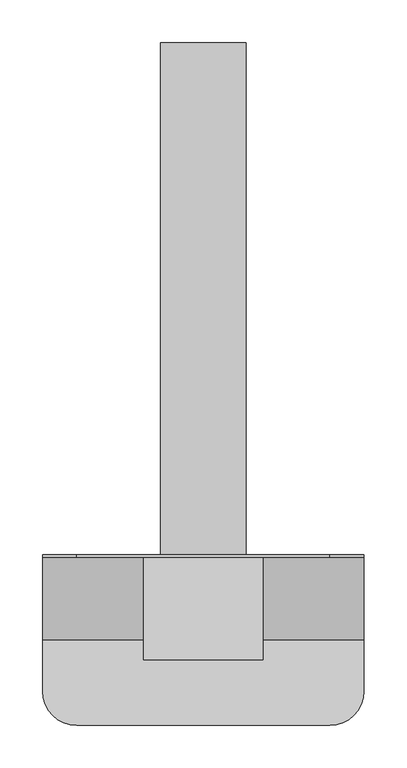
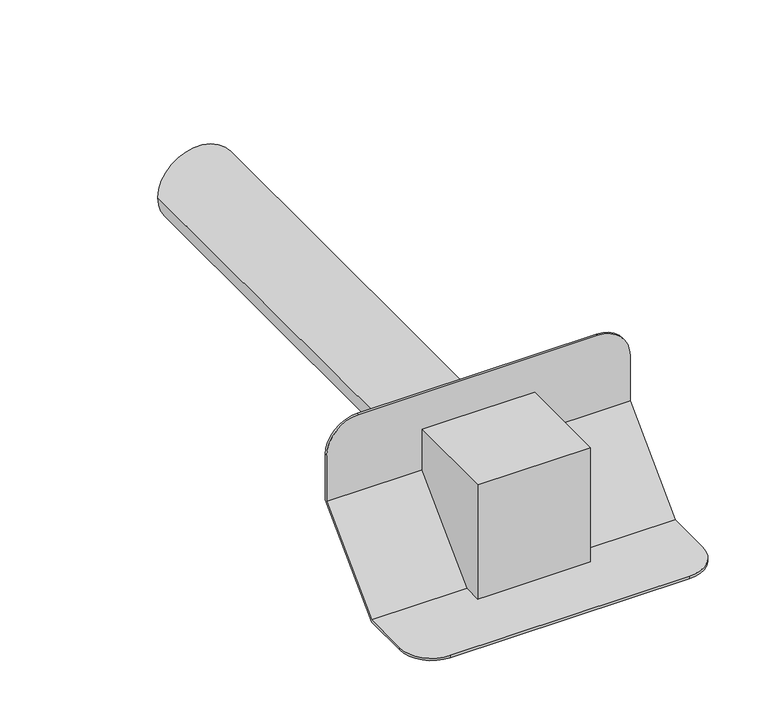
"""IFC4 building model written with IfcOpenShell, lengths in millimetres: proxy geometry, TN_Воронка парапетная ТехноНИКОЛЬ круглая_Тип 2 : Воронка парапетная ТехноНИКОЛЬ с галтелью 110х600."""

from ifc_helpers import new_model, si_unit, frame, origin, place, context, project, spatial, polyline, circle_curve, ellipse_curve, outline, extrude, source, transform, mapped, element, save
from ifc_brep_helpers import plane_surface, cylinder_surface, revolved_surface, advanced_brep


def specialty_equipment_09305b09(model_context):
    return source(origin(), model_context, "Body", "SolidModel", [
        extrude(outline(polyline([(-123.0, 3.0), (-123.0, 153.0), (-3.0, 153.0), (-3.0, 100.0), (-100.0, 3.0), (-123.0, 3.0)])), frame((-70.0, 0.0, 0.0), z_axis=(1.0, 0.0, 0.0), x_axis=(0.0, 1.0, 0.0)), (0.0, 0.0, 1.0), 140.0),
        advanced_brep(
        [(-188.5, -160.0, 3.0), (-148.5, -200.0, 3.0), (148.5, -200.0, 3.0), (188.5, -160.0, 3.0), (188.5, -100.0, 3.0), (-188.5, -100.0, 3.0), (-188.5, -160.0, 0.0), (-188.5, -100.0, 0.0), (188.5, -100.0, 0.0), (188.5, -160.0, 0.0), (148.5, -200.0, 0.0), (-148.5, -200.0, 0.0), (188.5, 0.0, 100.0), (188.5, 0.0, 160.0), (188.5, -3.0, 160.0), (188.5, -3.0, 100.0), (-188.5, -3.0, 100.0), (-188.5, -3.0, 160.0), (-188.5, 0.0, 160.0), (-188.5, 0.0, 100.0), (148.5, -3.0, 200.0), (-148.5, -3.0, 200.0), (-44.5421149, -3.0, 100.0), (44.5421149, -3.0, 100.0), (-148.5, 0.0, 200.0), (148.5, 0.0, 200.0), (47.6969601, 0.0, 100.0), (-47.6969601, 0.0, 100.0), (-50.0, 600.0, 85.0), (50.0, 600.0, 85.0), (-47.0, 600.0, 85.0), (47.0, 600.0, 85.0), (50.0, -15.0, 85.0), (-50.0, -15.0, 85.0), (47.0, -18.0, 85.0), (-47.0, -18.0, 85.0)],
        [
            (0, 1, circle_curve(frame((-148.5, -160.0, 3.0), z_axis=(0.0, 0.0, 1.0), x_axis=(1.0, 0.0, 0.0)), 40.0)),
            (1, 2),
            (2, 3, circle_curve(frame((148.5, -160.0, 3.0), z_axis=(0.0, 0.0, 1.0), x_axis=(1.0, 0.0, 0.0)), 40.0)),
            (3, 4),
            (4, 5),
            (5, 0),
            (6, 7),
            (7, 8),
            (8, 9),
            (9, 10, circle_curve(frame((148.5, -160.0, 0.0), z_axis=(0.0, 0.0, -1.0), x_axis=(1.0, 0.0, 0.0)), 40.0)),
            (10, 11),
            (11, 6, circle_curve(frame((-148.5, -160.0, 0.0), z_axis=(0.0, 0.0, -1.0), x_axis=(1.0, 0.0, 0.0)), 40.0)),
            (0, 6),
            (11, 1),
            (10, 2),
            (9, 3),
            (8, 12),
            (12, 13),
            (13, 14),
            (14, 15),
            (15, 4),
            (5, 16),
            (16, 17),
            (17, 18),
            (18, 19),
            (19, 7),
            (14, 20, circle_curve(frame((148.5, -3.0, 160.0), z_axis=(0.0, -1.0, 0.0), x_axis=(1.0, 0.0, 0.0)), 40.0)),
            (20, 21),
            (21, 17, circle_curve(frame((-148.5, -3.0, 160.0), z_axis=(0.0, -1.0, 0.0), x_axis=(1.0, 0.0, 0.0)), 40.0)),
            (16, 22),
            (22, 23, circle_curve(frame((0.0, -3.0, 85.0), z_axis=(0.0, 1.0, 0.0), x_axis=(1.0, 0.0, 0.0)), 47.0)),
            (23, 15),
            (18, 24, circle_curve(frame((-148.5, 0.0, 160.0), z_axis=(0.0, 1.0, 0.0), x_axis=(1.0, 0.0, 0.0)), 40.0)),
            (24, 25),
            (25, 13, circle_curve(frame((148.5, 0.0, 160.0), z_axis=(0.0, 1.0, 0.0), x_axis=(1.0, 0.0, 0.0)), 40.0)),
            (12, 26),
            (26, 27, circle_curve(frame((0.0, 0.0, 85.0), z_axis=(0.0, -1.0, 0.0), x_axis=(1.0, 0.0, 0.0)), 50.0)),
            (27, 19),
            (25, 20),
            (24, 21),
            (28, 29, circle_curve(frame((0.0, 600.0, 85.0), z_axis=(0.0, 1.0, 0.0), x_axis=(1.0, 0.0, 0.0)), 50.0)),
            (29, 28, circle_curve(frame((0.0, 600.0, 85.0), z_axis=(0.0, 1.0, 0.0), x_axis=(1.0, 0.0, 0.0)), 50.0)),
            (30, 31, circle_curve(frame((0.0, 600.0, 85.0), z_axis=(0.0, -1.0, 0.0), x_axis=(1.0, 0.0, 0.0)), 47.0)),
            (31, 30, circle_curve(frame((0.0, 600.0, 85.0), z_axis=(0.0, -1.0, 0.0), x_axis=(1.0, 0.0, 0.0)), 47.0)),
            (29, 32),
            (32, 33, ellipse_curve(frame((0.0, -15.0, 85.0), z_axis=(0.0, 0.7071067811865469, -0.7071067811865481), x_axis=(0.0, -0.7071067811865481, -0.7071067811865469)), 70.7106781, 50.0)),
            (33, 28),
            (33, 27, ellipse_curve(frame((0.0, -15.0, 85.0), z_axis=(0.0, 0.7071067811865469, -0.7071067811865481), x_axis=(0.0, -0.7071067811865481, -0.7071067811865469)), 70.7106781, 50.0)),
            (26, 32, ellipse_curve(frame((0.0, -15.0, 85.0), z_axis=(0.0, 0.7071067811865469, -0.7071067811865481), x_axis=(0.0, -0.7071067811865481, -0.7071067811865469)), 70.7106781, 50.0)),
            (31, 34),
            (34, 23, ellipse_curve(frame((0.0, -18.0, 85.0), z_axis=(0.0, -0.7071067811865469, 0.7071067811865482), x_axis=(0.0, 0.707106781186548, 0.7071067811865469)), 66.4680374, 47.0)),
            (22, 35, ellipse_curve(frame((0.0, -18.0, 85.0), z_axis=(0.0, -0.7071067811865469, 0.7071067811865482), x_axis=(0.0, 0.707106781186548, 0.7071067811865469)), 66.4680374, 47.0)),
            (35, 30),
            (35, 34, ellipse_curve(frame((0.0, -18.0, 85.0), z_axis=(0.0, -0.7071067811865469, 0.7071067811865482), x_axis=(0.0, 0.707106781186548, 0.7071067811865469)), 66.4680374, 47.0)),
        ],
        [
            plane_surface(frame((-108.5, -160.0, 3.0), z_axis=(0.0, 0.0, 1.0), x_axis=(0.0, 1.0, 0.0))),
            plane_surface(frame((-108.5, -160.0, 0.0), z_axis=(0.0, 0.0, -1.0), x_axis=(0.0, -1.0, 0.0))),
            cylinder_surface(frame((-148.5, -160.0, 0.0), z_axis=(0.0, 0.0, 1.0), x_axis=(1.0, 0.0, 0.0)), 40.0),
            plane_surface(frame((-148.5, -200.0, 3.0), z_axis=(0.0, -1.0, 0.0), x_axis=(0.0, 0.0, -1.0))),
            cylinder_surface(frame((148.5, -160.0, 0.0), z_axis=(0.0, 0.0, 1.0), x_axis=(1.0, 0.0, 0.0)), 40.0),
            plane_surface(frame((188.5, -160.0, 3.0), z_axis=(1.0, 0.0, 0.0), x_axis=(0.0, 0.0, -1.0))),
            plane_surface(frame((-188.5, -100.0, 3.0), z_axis=(-1.0, 0.0, 0.0), x_axis=(0.0, 0.0, -1.0))),
            plane_surface(frame((-188.5, -3.0, 100.0), z_axis=(0.0, -1.0, 0.0), x_axis=(1.0, 0.0, 0.0))),
            plane_surface(frame((-188.5, 0.0, 100.0), z_axis=(0.0, 1.0, 0.0), x_axis=(-1.0, 0.0, 0.0))),
            cylinder_surface(frame((148.5, 0.0, 160.0), z_axis=(0.0, -1.0, 0.0), x_axis=(1.0, 0.0, 0.0)), 40.0),
            plane_surface(frame((148.5, -3.0, 200.0), z_axis=(0.0, 0.0, 1.0), x_axis=(0.0, 1.0, 0.0))),
            cylinder_surface(frame((-148.5, 0.0, 160.0), z_axis=(0.0, -1.0, 0.0), x_axis=(1.0, 0.0, 0.0)), 40.0),
            plane_surface(frame((50.0, 600.0, 85.0), z_axis=(0.0, 1.0, 0.0), x_axis=(0.0, 0.0, -1.0))),
            cylinder_surface(frame((0.0, 600.0, 85.0), z_axis=(0.0, -1.0, 0.0), x_axis=(1.0, 0.0, 0.0)), 50.0),
            revolved_surface(polyline([(47.0, 600.0, 85.0), (47.0, -64.9999999777011, 85.0)]), (0.0, 0.0, 85.0), (0.0, 1.0, 0.0)),
            plane_surface(frame((188.5, -3.0, 100.0), z_axis=(0.0, -0.7071067811865469, 0.7071067811865482), x_axis=(-1.0, 0.0, 0.0))),
            plane_surface(frame((188.5, -100.0, 0.0), z_axis=(0.0, 0.7071067811865469, -0.7071067811865481), x_axis=(-1.0, 0.0, 0.0))),
        ],
        [
            (0, [[1, 2, 3, 4, 5, 6]]),
            (1, [[7, 8, 9, 10, 11, 12]]),
            (2, [[-1, 13, -12, 14]]),
            (3, [[-2, -14, -11, 15]]),
            (4, [[-3, -15, -10, 16]]),
            (5, [[-4, -16, -9, 17, 18, 19, 20, 21]]),
            (6, [[-6, 22, 23, 24, 25, 26, -7, -13]]),
            (7, [[-20, 27, 28, 29, -23, 30, 31, 32]]),
            (8, [[-25, 33, 34, 35, -18, 36, 37, 38]]),
            (9, [[-27, -19, -35, 39]]),
            (10, [[-28, -39, -34, 40]]),
            (11, [[-29, -40, -33, -24]]),
            (12, [[41, 42], [43, 44]]),
            (13, [[-42, 45, 46, 47]]),
            (13, [[-41, -47, 48, -37, 49, -45]]),
            (14, [[-44, 50, 51, -31, 52, 53]]),
            (14, [[-43, -53, 54, -50]]),
            (15, [[-21, -32, -51, -54, -52, -30, -22, -5]]),
            (16, [[-17, -8, -26, -38, -48, -46, -49, -36]]),
        ],
    ),
    ])


if __name__ == "__main__":
    model = new_model("IFC4")
    model_context = context("Model", 3, world=origin())
    ifc_project = project(units=[si_unit("LENGTHUNIT", "METRE", prefix="MILLI")], contexts=[model_context])
    site = spatial("IfcSite", under=ifc_project)
    building = spatial("IfcBuilding", under=site)
    placement = place(None, origin())
    specialty_equipment_shape = specialty_equipment_09305b09(model_context)
    element("IfcBuildingElementProxy", 1, Name="TN_Воронка парапетная ТехноНИКОЛЬ круглая_Тип 2 : Воронка парапетная ТехноНИКОЛЬ с галтелью 110х600", ObjectType="TN_Воронка парапетная ТехноНИКОЛЬ круглая_Тип 2 : Воронка парапетная ТехноНИКОЛЬ с галтелью 110х600", at=placement, inside=building, context=model_context, shape_type="MappedRepresentation", body=[
        mapped(specialty_equipment_shape, transform((0.0, 0.0, 0.0), x_axis=(1.0, 0.0, 0.0), y_axis=(0.0, 1.0, 0.0), z_axis=(0.0, 0.0, 1.0))),
    ])
    save(model, "model.ifc")

# Revit data of these elements
# Type "TN_Воронка парапетная ТехноНИКОЛЬ круглая_Тип 2 : Воронка парапетная ТехноНИКОЛЬ с галтелью 110х600"
#   Description = "Воронка предназначена для организации внешнего водостока через балконы и парапеты на пониженных участках кровли. Также воронка может являться парапетным переливом, которая устанавливается в случаях аварийного сброса воды при засорении основной воронки внутреннего водостока. Воронки комплектуются листвоуловителем и имеют сформированную галтель размером 100ммх100мм, что облегчает монтаж битумной гидроизоляции в данном узле и повышает его надежность при эксплуатации.\r\nСоединение с водосточной системой осуществляется через угловые отводы."
#   Manufacturer = "ТехноНИКОЛЬ"
#   ADSK_Примечание = ""
#   ADSK_Обозначение = "ТехноНИКОЛЬ"
#   ADSK_Наименование = "Воронка парапетная ТехноНИКОЛЬ с галтелью 110х600"
#   ADSK_Марка = ""
#   ADSK_Код изделия = "69752"
#   ADSK_Завод-изготовитель = "ТехноНИКОЛЬ"
#   ADSK_Единица измерения = "шт."
#   ADSK_Группирование = "Комплектующие и воронки"
#   ADSK_URL страницы изделия = ""
#   ADSK_URL документации изделия = ""
#   Ширина фланца = 377 mm
#   Размер фланца по вертикали = 200 mm
#   Длина расчетная [instance default] = 600 mm
#   Длина отвода [instance default] = 600 mm
#   Размер фланца по горизонтали = 200 mm
#   ADSK_Количество = 1
#   Видимость_Переход [instance default] = no
#   Видимость_Листоуловитель [instance default] = no
#   Материал = TN_ПВХ_Черный
#   Default Elevation = 0
#   URL = ""
# Element 1 (IfcBuildingElementProxy, "TN_Воронка парапетная ТехноНИКОЛЬ круглая_Тип 2 : Воронка парапетная ТехноНИКОЛЬ с галтелью 110х600")
#   Видимость_Переход = yes
#   Видимость_Листоуловитель = yes
#   Materials on its faces: "TN_ПВХ_Черный"
# Materials
#   "TN_ПВХ_Черный": class "Типовые", colour RGB 48 48 48, transparency 0, Cost = 0
